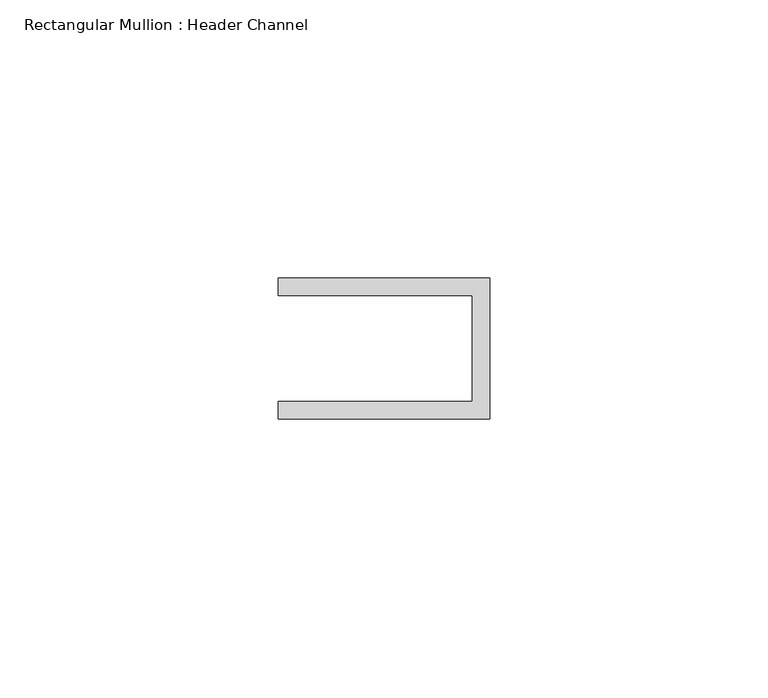
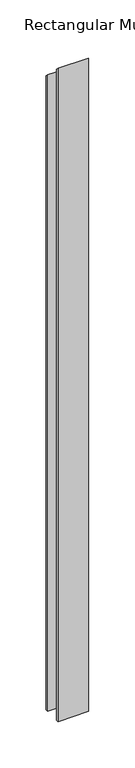
"""IFC4 building model written with IfcOpenShell, lengths in millimetres: member geometry, Rectangular Mullion : Header Channel."""

from ifc_helpers import new_model, si_unit, origin, place, context, project, spatial, faceted_brep, source, transform, mapped, element, save


def rectangular_mullion_header_channel_3a661f62(model_context):
    return source(origin(), model_context, "Body", "Brep", [
        faceted_brep([(0.0, -12.7, -845.4185498), (-38.1, -12.7, -845.4185498), (-38.1, -9.525, -845.4185498), (-3.175, -9.525, -845.4185498), (-3.175, 9.525, -845.4185498), (-38.1, 9.525, -845.4185498), (-38.1, 12.7, -845.4185498), (0.0, 12.7, -845.4185498), (0.0, 12.7, -12.7), (0.0, -12.7, 12.7), (-38.1, 12.7, -12.7), (-38.1, 9.525, -9.525), (-3.175, 9.525, -9.525), (-3.175, -9.525, 9.525), (-38.1, -9.525, 9.525), (-38.1, -12.7, 12.7)], [[[0, 1, 2, 3, 4, 5, 6, 7]], [[8, 9, 0, 7]], [[10, 8, 7, 6]], [[11, 10, 6, 5]], [[12, 11, 5, 4]], [[13, 12, 4, 3]], [[14, 13, 3, 2]], [[15, 14, 2, 1]], [[9, 15, 1, 0]], [[9, 8, 10, 11, 12, 13, 14, 15]]]),
    ])


if __name__ == "__main__":
    model = new_model("IFC4")
    model_context = context("Model", 3, world=origin())
    ifc_project = project(units=[si_unit("LENGTHUNIT", "METRE", prefix="MILLI")], contexts=[model_context])
    site = spatial("IfcSite", under=ifc_project)
    building = spatial("IfcBuilding", under=site)
    placement = place(None, origin())
    rectangular_mullion_header_channel_shape = rectangular_mullion_header_channel_3a661f62(model_context)
    element("IfcMember", 1, ObjectType="Rectangular Mullion : Header Channel", at=placement, inside=building, context=model_context, shape_type="MappedRepresentation", body=[
        mapped(rectangular_mullion_header_channel_shape, transform((0.0, 0.0, 0.0), x_axis=(1.0, 0.0, 0.0), y_axis=(0.0, 1.0, 0.0), z_axis=(0.0, 0.0, 1.0))),
    ])
    save(model, "model.ifc")

# Revit data of these elements
# Type "Rectangular Mullion : Header Channel"
#   built-in parameter 1007322 = 0.0833333 (stored number, unit not read)
#   built-in parameter 1007321 = -0.03125 (stored number, unit not read)
#   built-in parameter 1007320 = 0.0416667 (stored number, unit not read)
# Element 1 (IfcMember, "Rectangular Mullion : Header Channel")
#   Materials on its faces: "ALUM"
# Materials
#   "ALUM": class "Generic", colour RGB 157 157 157, transparency 0, Cost = 0
